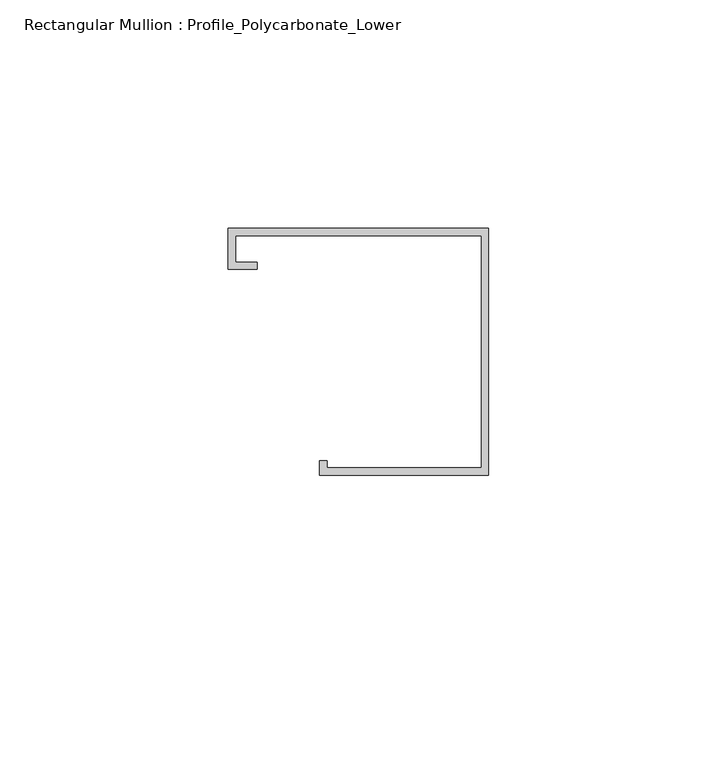
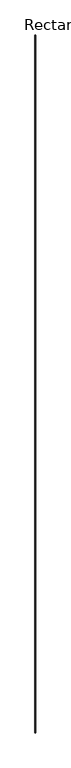
"""IFC4 building model written with IfcOpenShell, lengths in millimetres: member geometry, Rectangular Mullion : Profile_Polycarbonate_Lower."""

import ifcopenshell
import ifcopenshell.guid

model = None  # the IFC model being written
_history = None  # IfcOwnerHistory: only IFC2X3 demands one
_inside = {}  # id of a spatial element -> (the spatial element, [elements in it])
_under = {}  # id of a project, library or spatial element -> (it, [spatial elements below it])
_declared = {}  # id of a project -> (the project, [libraries it declares])
_typed = {}  # id of a type object -> (the type object, [elements of that type])
_made_of = {}  # id of a material, layer set ... -> (it, [elements and type objects made of it])


def new_model(schema):
    """Start an empty IFC model of exactly this schema.

    Asked for "IFC4X3", IfcOpenShell would pick the latest addendum, in which some entities
    have other attributes; the version numbers below select the first issue.
    IFC2X3 requires an IfcOwnerHistory on every rooted entity: one is made here for all.
    """
    global model, _history
    if schema == "IFC4X3":
        model = ifcopenshell.file(schema_version=(4, 3, 0, 0))
    else:
        model = ifcopenshell.file(schema=schema)
    _inside.clear()
    _under.clear()
    _declared.clear()
    _typed.clear()
    _made_of.clear()
    _history = None
    if model.schema == "IFC2X3":
        org = make("IfcOrganization", Name="unknown")
        user = make(
            "IfcPersonAndOrganization",
            ThePerson=make("IfcPerson", FamilyName="unknown"),
            TheOrganization=org,
        )
        app = make(
            "IfcApplication",
            ApplicationDeveloper=org,
            Version="unknown",
            ApplicationFullName="unknown",
            ApplicationIdentifier="unknown",
        )
        _history = make(
            "IfcOwnerHistory",
            OwningUser=user,
            OwningApplication=app,
            ChangeAction="ADDED",
            CreationDate=0,
        )
    return model


def make(cls, **values):
    """One entity of the class cls with the attributes given. An attribute that is None is left unset."""
    return model.create_entity(
        cls, **{name: value for name, value in values.items() if value is not None}
    )


def rooted(cls, **values):
    """An entity with a GlobalId (a new one), such as an element, a storey or a relation."""
    return make(cls, GlobalId=ifcopenshell.guid.new(), OwnerHistory=_history, **values)


def si_unit(unit_type, name, prefix=None):
    """IfcSIUnit, for example si_unit("LENGTHUNIT", "METRE", prefix="MILLI")."""
    return make("IfcSIUnit", UnitType=unit_type, Prefix=prefix, Name=name)


def assignment(units):
    """IfcUnitAssignment: the units of a project."""
    return None if units is None else make("IfcUnitAssignment", Units=units)


def point(xyz):
    """IfcCartesianPoint."""
    return None if xyz is None else make("IfcCartesianPoint", Coordinates=xyz)


def direction(xyz):
    """IfcDirection."""
    return None if xyz is None else make("IfcDirection", DirectionRatios=xyz)


def frame(location, z_axis=None, x_axis=None):
    """IfcAxis2Placement3D, a coordinate frame: its origin and axes. An axis left out is left unset."""
    return make(
        "IfcAxis2Placement3D",
        Location=point(location),
        Axis=direction(z_axis),
        RefDirection=direction(x_axis),
    )


def origin():
    """The frame at (0, 0, 0) with its axes left unset."""
    return frame((0.0, 0.0, 0.0))


def place(relative_to, where):
    """IfcLocalPlacement: puts the frame where relative to a parent placement (None: the world)."""
    return make(
        "IfcLocalPlacement", PlacementRelTo=relative_to, RelativePlacement=where
    )


def context(
    kind, dimensions, precision=None, world=None, true_north=None, identifier=None
):
    """IfcGeometricRepresentationContext, for example the 3D "Model" context."""
    return make(
        "IfcGeometricRepresentationContext",
        ContextIdentifier=identifier,
        ContextType=kind,
        CoordinateSpaceDimension=dimensions,
        Precision=precision,
        WorldCoordinateSystem=world,
        TrueNorth=true_north,
    )


def project(units=None, contexts=None):
    """IfcProject with its units and contexts."""
    return rooted(
        "IfcProject",
        Name="project",
        RepresentationContexts=contexts,
        UnitsInContext=assignment(units),
    )


def spatial(cls, under=None, at=None, **own):
    """A site, building, storey or space (cls), placed at a placement, below another one or the project."""
    s = rooted(cls, ObjectPlacement=at, **own)
    if under is not None:
        _under.setdefault(under.id(), (under, []))[1].append(s)
    return s


def polyline(points):
    """IfcPolyline through the points."""
    return make("IfcPolyline", Points=[point(p) for p in points])


def outline(outer, holes=None, kind="AREA"):
    """IfcArbitraryClosedProfileDef: a profile drawn as a closed curve; with holes, ...WithVoids."""
    if holes is None:
        return make("IfcArbitraryClosedProfileDef", ProfileType=kind, OuterCurve=outer)
    return make(
        "IfcArbitraryProfileDefWithVoids",
        ProfileType=kind,
        OuterCurve=outer,
        InnerCurves=holes,
    )


def extrude(swept, where, along, depth):
    """IfcExtrudedAreaSolid: the profile swept, set in the frame where, extruded along a direction by depth."""
    return make(
        "IfcExtrudedAreaSolid",
        SweptArea=swept,
        Position=where,
        ExtrudedDirection=direction(along),
        Depth=depth,
    )


def shape(context_of_items, identifier, shape_type, items):
    """IfcShapeRepresentation: the items that make up one representation, for example the "Body"."""
    return make(
        "IfcShapeRepresentation",
        ContextOfItems=context_of_items,
        RepresentationIdentifier=identifier,
        RepresentationType=shape_type,
        Items=items,
    )


def source(mapping_origin, context_of_items, identifier, shape_type, items):
    """IfcRepresentationMap: a shape defined once, which mapped items show again and again."""
    return make(
        "IfcRepresentationMap",
        MappingOrigin=mapping_origin,
        MappedRepresentation=shape(context_of_items, identifier, shape_type, items),
    )


def transform(
    local_origin,
    x_axis=None,
    y_axis=None,
    z_axis=None,
    scale=None,
    scale2=None,
    scale3=None,
    uniform=True,
):
    """IfcCartesianTransformationOperator3D, or its non-uniform kind. x_axis, y_axis, z_axis: its Axis1, 2, 3."""
    if uniform:
        return make(
            "IfcCartesianTransformationOperator3D",
            Axis1=direction(x_axis),
            Axis2=direction(y_axis),
            LocalOrigin=point(local_origin),
            Scale=scale,
            Axis3=direction(z_axis),
        )
    return make(
        "IfcCartesianTransformationOperator3DnonUniform",
        Axis1=direction(x_axis),
        Axis2=direction(y_axis),
        LocalOrigin=point(local_origin),
        Scale=scale,
        Axis3=direction(z_axis),
        Scale2=scale2,
        Scale3=scale3,
    )


def mapped(mapping_source, mapping_target):
    """IfcMappedItem: shows the shape of a source again, moved by a transform."""
    return make(
        "IfcMappedItem", MappingSource=mapping_source, MappingTarget=mapping_target
    )


def made_of(thing, what):
    """Note that an element or type object is made of a material, layer set ...; save() writes the relation."""
    if what is not None:
        _made_of.setdefault(what.id(), (what, []))[1].append(thing)
    return thing


def element(
    cls,
    number,
    at=None,
    inside=None,
    cuts=None,
    type_object=None,
    material=None,
    context=None,
    identifier="Body",
    shape_type=None,
    held_by="IfcProductDefinitionShape",
    body=None,
    shapes=None,
    **own,
):
    """One element of the class cls, such as IfcWall. Its Tag is "e" and its number.

    at: its placement. inside: the storey or other place that contains it. cuts: it is an
    opening in that element (IfcRelVoidsElement). A single representation is given by context,
    identifier, shape_type and body (its items); several are given by shapes. held_by: the class
    of the entity that holds the representations. save() writes the other relations.
    """
    e = rooted(cls, Tag="e%d" % number, ObjectPlacement=at, **own)
    if body is not None:
        shapes = [shape(context, identifier, shape_type, body)]
    if shapes is not None:
        e.Representation = make(held_by, Representations=shapes)
    if inside is not None:
        _inside.setdefault(inside.id(), (inside, []))[1].append(e)
    if cuts is not None:
        rooted(
            "IfcRelVoidsElement", RelatingBuildingElement=cuts, RelatedOpeningElement=e
        )
    if type_object is not None:
        _typed.setdefault(type_object.id(), (type_object, []))[1].append(e)
    return made_of(e, material)


def aggregate(whole, parts):
    """IfcRelAggregates: a whole, such as a stair, and the parts it consists of."""
    return rooted("IfcRelAggregates", RelatingObject=whole, RelatedObjects=parts)


def save(model, path):
    """Write the relations noted so far, then the file.

    IfcRelAggregates (storeys below a building ...), IfcRelContainedInSpatialStructure (elements
    in a storey), IfcRelDefinesByType, IfcRelAssociatesMaterial and IfcRelDeclares: one each for
    every whole, place, type object, material and project.
    """
    for whole, parts in _under.values():
        aggregate(whole, parts)
    for where, things in _inside.values():
        rooted(
            "IfcRelContainedInSpatialStructure",
            RelatedElements=things,
            RelatingStructure=where,
        )
    for kind, things in _typed.values():
        rooted("IfcRelDefinesByType", RelatedObjects=things, RelatingType=kind)
    for what, things in _made_of.values():
        rooted("IfcRelAssociatesMaterial", RelatedObjects=things, RelatingMaterial=what)
    for by, libraries in _declared.values():
        rooted("IfcRelDeclares", RelatingContext=by, RelatedDefinitions=libraries)
    model.write(path)


def rectangular_mullion_profile_polycarbonate_lower_af46c414(model_context):
    return source(origin(), model_context, "Body", "SweptSolid", [
        extrude(outline(polyline([(0.0, 28.984575), (0.0, -25.015825), (-36.9824, -25.015825), (-36.9824, -21.840825), (-35.3949, -21.840825), (-35.3949, -23.428325), (-1.5875, -23.428325), (-1.5875, 27.397075), (-55.4101, 27.397075), (-55.4101, 21.580475), (-50.6476, 21.580475), (-50.6476, 19.992975), (-56.9976, 19.992975), (-56.9976, 28.984575), (0.0, 28.984575)])), frame((0.0, 0.0, -80941.7668531), z_axis=(0.0, 0.0, 1.0), x_axis=(1.0, 0.0, 0.0)), (0.0, 0.0, 1.0), 80941.7668531),
    ])


if __name__ == "__main__":
    model = new_model("IFC4")
    model_context = context("Model", 3, world=origin())
    ifc_project = project(units=[si_unit("LENGTHUNIT", "METRE", prefix="MILLI")], contexts=[model_context])
    site = spatial("IfcSite", under=ifc_project)
    building = spatial("IfcBuilding", under=site)
    placement = place(None, origin())
    rectangular_mullion_profile_polycarbonate_lower_shape = rectangular_mullion_profile_polycarbonate_lower_af46c414(model_context)
    element("IfcMember", 1, ObjectType="Rectangular Mullion : Profile_Polycarbonate_Lower", at=placement, inside=building, context=model_context, shape_type="MappedRepresentation", body=[
        mapped(rectangular_mullion_profile_polycarbonate_lower_shape, transform((0.0, 0.0, 0.0), x_axis=(1.0, 0.0, 0.0), y_axis=(0.0, 1.0, 0.0), z_axis=(0.0, 0.0, 1.0))),
    ])
    save(model, "model.ifc")

# Revit data of these elements
# Type "Rectangular Mullion : Profile_Polycarbonate_Lower"
#   built-in parameter 1007322 = 0.177167 (stored number, unit not read)
#   built-in parameter 1007321 = 0 (stored number, unit not read)
#   built-in parameter 1007320 = 0.00520833 (stored number, unit not read)
